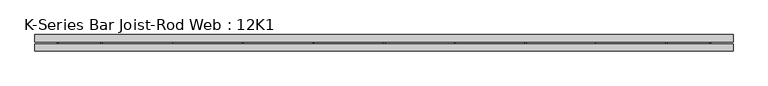
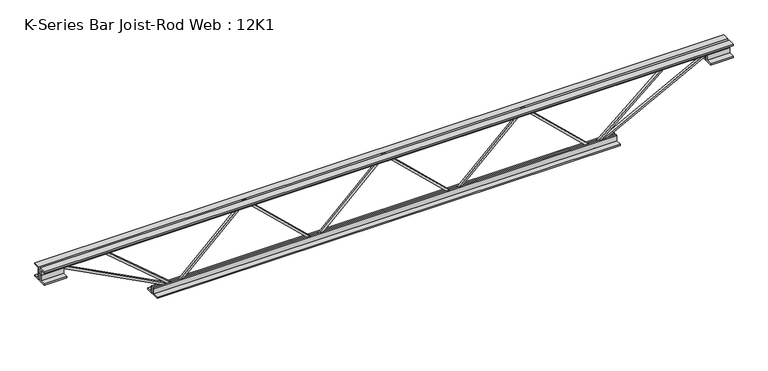
"""IFC4 building model written with IfcOpenShell, lengths in millimetres: beam geometry, K-Series Bar Joist-Rod Web : 12K1."""

from ifc_helpers import new_model, si_unit, frame, origin, place, context, project, spatial, polyline, outline, extrude, source, transform, mapped, element, save


def k_series_bar_joist_rod_web_12k1_474d8b97(model_context):
    return source(origin(), model_context, "Body", "SweptSolid", [
        extrude(outline(polyline([(-141.2875, -313.53125), (-150.8125, -313.53125), (-150.8125, -308.45339), (141.2875, -1.27214), (141.2875, 1.27214), (-150.8125, 308.45339), (-150.8125, 313.53125), (-141.2875, 313.53125), (-141.2875, 312.25911), (150.8125, 5.07786), (150.8125, -5.07786), (-141.2875, -312.25911), (-141.2875, -313.53125)])), frame((0.0, -4.7625, 0.0), z_axis=(0.0, 1.0, 0.0), x_axis=(0.0, 0.0, 1.0)), (0.0, 0.0, 1.0), 9.525),
        extrude(outline(polyline([(-141.2875, 313.53125), (-150.8125, 313.53125), (-150.8125, 318.60911), (141.2875, 625.79036), (141.2875, 628.33464), (-150.8125, 935.51589), (-150.8125, 940.59375), (-141.2875, 940.59375), (-141.2875, 939.32161), (150.8125, 632.14036), (150.8125, 621.98464), (-141.2875, 314.80339), (-141.2875, 313.53125)])), frame((0.0, -4.7625, 0.0), z_axis=(0.0, 1.0, 0.0), x_axis=(0.0, 0.0, 1.0)), (0.0, 0.0, 1.0), 9.525),
        extrude(outline(polyline([(-141.2875, -940.59375), (-150.8125, -940.59375), (-150.8125, -935.51589), (141.2875, -628.33464), (141.2875, -625.79036), (-150.8125, -318.60911), (-150.8125, -313.53125), (-141.2875, -313.53125), (-141.2875, -314.80339), (150.8125, -621.98464), (150.8125, -632.14036), (-141.2875, -939.32161), (-141.2875, -940.59375)])), frame((0.0, -4.7625, 0.0), z_axis=(0.0, 1.0, 0.0), x_axis=(0.0, 0.0, 1.0)), (0.0, 0.0, 1.0), 9.525),
        extrude(outline(polyline([(4.7625, 152.4), (36.5125, 152.4), (36.5125, 146.05), (11.1125, 146.05), (11.1125, 120.65), (4.7625, 120.65), (4.7625, 152.4)])), frame((-1550.19375, 0.0, 0.0), z_axis=(1.0, 0.0, 0.0), x_axis=(0.0, 1.0, 0.0)), (0.0, 0.0, 1.0), 3100.3875),
        extrude(outline(polyline([(-4.7625, 152.4), (-4.7625, 120.65), (-11.1125, 120.65), (-11.1125, 146.05), (-36.5125, 146.05), (-36.5125, 152.4), (-4.7625, 152.4)])), frame((-1550.19375, 0.0, 0.0), z_axis=(1.0, 0.0, 0.0), x_axis=(0.0, 1.0, 0.0)), (0.0, 0.0, 1.0), 3100.3875),
        extrude(outline(polyline([(-4.7625, 88.9), (-36.5125, 88.9), (-36.5125, 95.25), (-11.1125, 95.25), (-11.1125, 120.65), (-4.7625, 120.65), (-4.7625, 88.9)])), frame((-1550.19375, 0.0, 0.0), z_axis=(1.0, 0.0, 0.0), x_axis=(0.0, 1.0, 0.0)), (0.0, 0.0, 1.0), 101.6),
        extrude(outline(polyline([(36.5125, 88.9), (4.7625, 88.9), (4.7625, 120.65), (11.1125, 120.65), (11.1125, 95.25), (36.5125, 95.25), (36.5125, 88.9)])), frame((-1550.19375, 0.0, 0.0), z_axis=(1.0, 0.0, 0.0), x_axis=(0.0, 1.0, 0.0)), (0.0, 0.0, 1.0), 101.6),
        extrude(outline(polyline([(4.7625, 88.9), (4.7625, 120.65), (11.1125, 120.65), (11.1125, 95.25), (36.5125, 95.25), (36.5125, 88.9), (4.7625, 88.9)])), frame((1448.59375, 0.0, 0.0), z_axis=(1.0, 0.0, 0.0), x_axis=(0.0, 1.0, 0.0)), (0.0, 0.0, 1.0), 101.6),
        extrude(outline(polyline([(-4.7625, 88.9), (-36.5125, 88.9), (-36.5125, 95.25), (-11.1125, 95.25), (-11.1125, 120.65), (-4.7625, 120.65), (-4.7625, 88.9)])), frame((1448.59375, 0.0, 0.0), z_axis=(1.0, 0.0, 0.0), x_axis=(0.0, 1.0, 0.0)), (0.0, 0.0, 1.0), 101.6),
        extrude(outline(polyline([(4.7625, -152.4), (4.7625, -120.65), (11.1125, -120.65), (11.1125, -146.05), (36.5125, -146.05), (36.5125, -152.4), (4.7625, -152.4)])), frame((-1042.19375, 0.0, 0.0), z_axis=(1.0, 0.0, 0.0), x_axis=(0.0, 1.0, 0.0)), (0.0, 0.0, 1.0), 2084.3875),
        extrude(outline(polyline([(-4.7625, -152.4), (-36.5125, -152.4), (-36.5125, -146.05), (-11.1125, -146.05), (-11.1125, -120.65), (-4.7625, -120.65), (-4.7625, -152.4)])), frame((-1042.19375, 0.0, 0.0), z_axis=(1.0, 0.0, 0.0), x_axis=(0.0, 1.0, 0.0)), (0.0, 0.0, 1.0), 2084.3875),
        extrude(outline(polyline([(0.0, -9.525), (0.0, 0.0), (573.7533355, 0.0), (573.7533355, -9.525), (0.0, -9.525)])), frame((-1450.8075214, 4.7625, 116.4332925), z_axis=(0.46483389898951377, 0.0, 0.885397902838157), x_axis=(0.885397902838157, 0.0, -0.46483389898951377)), (0.0, 0.0, 1.0), 9.525),
        extrude(outline(polyline([(0.0, -9.525), (0.0, 0.0), (411.6196481, 0.0), (411.6196481, -9.525), (0.0, -9.525)])), frame((-1257.2107583, 4.7625, 117.0223972), z_axis=(0.6479282541820981, 0.0, 0.7617013702446246), x_axis=(0.7617013702446246, 0.0, -0.6479282541820981)), (0.0, 0.0, 1.0), 9.525),
        extrude(outline(polyline([(0.0, -9.525), (0.0, 0.0), (573.7533355, 0.0), (573.7533355, -9.525), (0.0, -9.525)])), frame((1450.8075214, -4.7625, 116.4332925), z_axis=(-0.46483389898949395, 0.0, 0.8853979028381674), x_axis=(-0.8853979028381674, 0.0, -0.46483389898949395)), (0.0, 0.0, 1.0), 9.525),
        extrude(outline(polyline([(0.0, -9.525), (0.0, 0.0), (411.6196481, 0.0), (411.6196481, -9.525), (0.0, -9.525)])), frame((1257.2107583, -4.7625, 117.0223972), z_axis=(-0.6479282541820912, 0.0, 0.7617013702446305), x_axis=(-0.7617013702446305, 0.0, -0.6479282541820912)), (0.0, 0.0, 1.0), 9.525),
    ])


if __name__ == "__main__":
    model = new_model("IFC4")
    model_context = context("Model", 3, world=origin())
    ifc_project = project(units=[si_unit("LENGTHUNIT", "METRE", prefix="MILLI")], contexts=[model_context])
    site = spatial("IfcSite", under=ifc_project)
    building = spatial("IfcBuilding", under=site)
    placement = place(None, origin())
    k_series_bar_joist_rod_web_12k1_shape = k_series_bar_joist_rod_web_12k1_474d8b97(model_context)
    element("IfcBeam", 1, ObjectType="K-Series Bar Joist-Rod Web : 12K1", at=placement, inside=building, context=model_context, shape_type="MappedRepresentation", body=[
        mapped(k_series_bar_joist_rod_web_12k1_shape, transform((0.0, 0.0, 0.0), x_axis=(1.0, 0.0, 0.0), y_axis=(0.0, 1.0, 0.0), z_axis=(0.0, 0.0, 1.0))),
    ])
    save(model, "model.ifc")

# Revit data of these elements
# Type "K-Series Bar Joist-Rod Web : 12K1"
#   Assembly Code = "B1010350"
#   Wt = 5
#   Web Thickness = 0' - 0 3/8"
#   Start Offset [instance default] = 0' - 0"
#   Start Extension [instance default] = 0' - 0"
#   Seat Length = 0' - 4"
#   Seat Depth = 0' - 2 1/2"
#   PanelArrayLength [instance default] = 20' - 0"
#   Panel [instance default] = 2' - 0"
#   End Offset [instance default] = 0' - 0"
#   End Extension [instance default] = 0' - 0"
#   End Panel = 2' - 0"
#   Cord Leg = 0' - 1 1/4"
#   Chord Thickness = 0' - 0 1/4"
#   Length [instance default] = 24' - 0"
#   Depth = 1' - 0"
#   PanelArrayNum [instance default] = 10
#   Structural Material = none
# Element 1 (IfcBeam, "K-Series Bar Joist-Rod Web : 12K1")
#   PanelArrayLength = 6' - 2 1/16"
#   Panel = 2' - 0 11/16"
#   PanelArrayNum = 3
